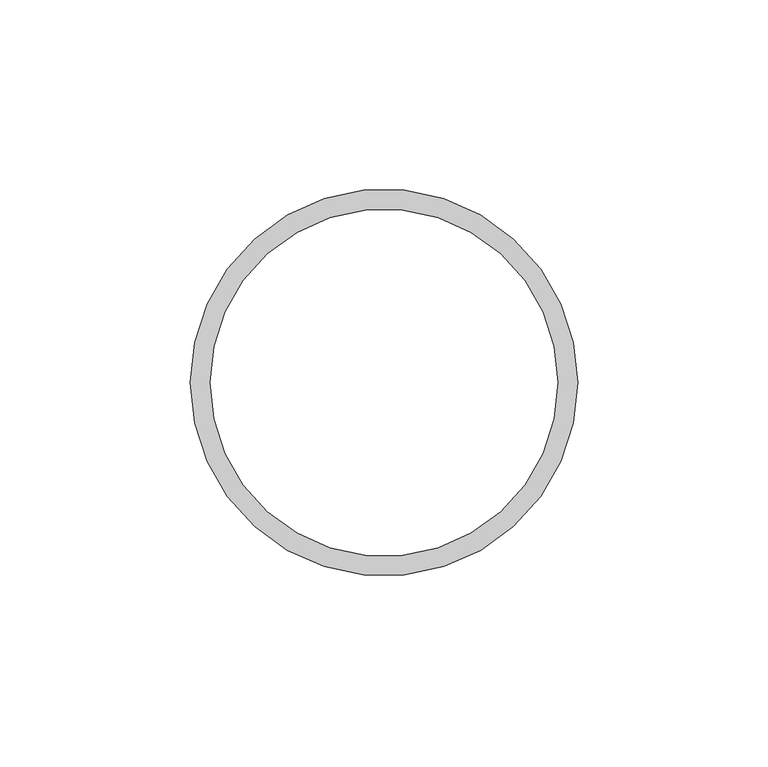
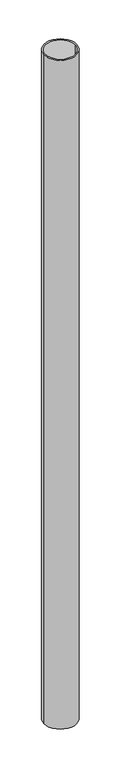
"""IFC4 building model written with IfcOpenShell, lengths in millimetres: proxy geometry, Generic Models 7:Generic Models 1:3:Generic Models 1:3 : Generic Models 7:Generic Models 1:305549:3:Generic Models 1:3:Generic Models 1:3 : Generic Models 7:Generic Models 1:305549:3 : Generic Models 7:Generic Models 1:3:Generic Models 1:3 : Generic Models 7:Generic Models 1:305549:301244:28 : Generic Models 7:Generic Models 1:3:Generic Models 1:3 : Generic Models 7:Generic Models 1:305549:3:Generic Models 1:3:Generic Models 1:3 : Generic Models 7:Generic Models 1:305549:3 : Generic Models 7:Generic Models 1:3:Generic Models 1:3 : Generic Models 7:Generic Models 1:305549:301244:308848."""

from ifc_helpers import new_model, si_unit, point, frame, frame_2d, origin, place, context, project, spatial, circle_curve, trimmed, segment, composite_curve, outline, extrude, source, transform, mapped, element, save


def generic_models_a17a7060(model_context):
    return source(origin(), model_context, "Body", "SweptSolid", [
        extrude(outline(composite_curve([segment(trimmed(circle_curve(frame_2d((560568.8617239, -572593.5413841)), 50.8), [point((560518.0617239, -572593.5413841))], [point((560619.6617239, -572593.5413841))], False, "CARTESIAN"), True, "CONTINUOUS"), segment(trimmed(circle_curve(frame_2d((560568.8617239, -572593.5413841)), 50.8), [point((560619.6617239, -572593.5413841))], [point((560518.0617239, -572593.5413841))], False, "CARTESIAN"), True, "CONTINUOUS")], self_intersect=False), holes=[composite_curve([segment(trimmed(circle_curve(frame_2d((560568.8617239, -572593.5413841)), 45.593), [point((560523.2687239, -572593.5413841))], [point((560614.4547239, -572593.5413841))], True, "CARTESIAN"), True, "CONTINUOUS"), segment(trimmed(circle_curve(frame_2d((560568.8617239, -572593.5413841)), 45.593), [point((560614.4547239, -572593.5413841))], [point((560523.2687239, -572593.5413841))], True, "CARTESIAN"), True, "CONTINUOUS")], self_intersect=False)]), frame((0.0, 0.0, 3929.0269064), z_axis=(0.0, 0.0, 1.0), x_axis=(1.0, 0.0, 0.0)), (0.0, 0.0, 1.0), 2205.0730936),
    ])


if __name__ == "__main__":
    model = new_model("IFC4")
    model_context = context("Model", 3, world=origin())
    ifc_project = project(units=[si_unit("LENGTHUNIT", "METRE", prefix="MILLI")], contexts=[model_context])
    site = spatial("IfcSite", under=ifc_project)
    building = spatial("IfcBuilding", under=site)
    placement = place(None, origin())
    generic_models_shape = generic_models_a17a7060(model_context)
    element("IfcBuildingElementProxy", 1, Name="Generic Models 7:Generic Models 1:3:Generic Models 1:3 : Generic Models 7:Generic Models 1:305549:3:Generic Models 1:3:Generic Models 1:3 : Generic Models 7:Generic Models 1:305549:3 : Generic Models 7:Generic Models 1:3:Generic Models 1:3 : Generic Models 7:Generic Models 1:305549:301244:28 : Generic Models 7:Generic Models 1:3:Generic Models 1:3 : Generic Models 7:Generic Models 1:305549:3:Generic Models 1:3:Generic Models 1:3 : Generic Models 7:Generic Models 1:305549:3 : Generic Models 7:Generic Models 1:3:Generic Models 1:3 : Generic Models 7:Generic Models 1:305549:301244:308848", ObjectType="Generic Models 7:Generic Models 1:3:Generic Models 1:3 : Generic Models 7:Generic Models 1:305549:3:Generic Models 1:3:Generic Models 1:3 : Generic Models 7:Generic Models 1:305549:3 : Generic Models 7:Generic Models 1:3:Generic Models 1:3 : Generic Models 7:Generic Models 1:305549:301244:28 : Generic Models 7:Generic Models 1:3:Generic Models 1:3 : Generic Models 7:Generic Models 1:305549:3:Generic Models 1:3:Generic Models 1:3 : Generic Models 7:Generic Models 1:305549:3 : Generic Models 7:Generic Models 1:3:Generic Models 1:3 : Generic Models 7:Generic Models 1:305549:301244:308848", at=placement, inside=building, context=model_context, shape_type="MappedRepresentation", body=[
        mapped(generic_models_shape, transform((0.0, 0.0, 0.0), x_axis=(1.0, 0.0, 0.0), y_axis=(0.0, 1.0, 0.0), z_axis=(0.0, 0.0, 1.0))),
    ])
    save(model, "model.ifc")

# Revit data of these elements
# Type "Generic Models 7:Generic Models 1:3:Generic Models 1:3 : Generic Models 7:Generic Models 1:305549:3:Generic Models 1:3:Generic Models 1:3 : Generic Models 7:Generic Models 1:305549:3 : Generic Models 7:Generic Models 1:3:Generic Models 1:3 : Generic Models 7:Generic Models 1:305549:301244:28 : Generic Models 7:Generic Models 1:3:Generic Models 1:3 : Generic Models 7:Generic Models 1:305549:3:Generic Models 1:3:Generic Models 1:3 : Generic Models 7:Generic Models 1:305549:3 : Generic Models 7:Generic Models 1:3:Generic Models 1:3 : Generic Models 7:Generic Models 1:305549:301244:308848"
#   NameOverride = "Generic Models 7:Generic Models 1:3:Generic Models 1:3 : Generic Models 7:Generic Models 1:305549:3:Generic Models 1:3:Generic Models 1:3 : Generic Models 7:Generic Models 1:305549:3 : Generic Models 7:Generic Models 1:3:Generic Models 1:3 : Generic Models 7:Generic Models 1:305549:301244:308848"
#   ObjectTypeOverride = "Generic Models 1:3:Generic Models 1:3 : Generic Models 7:Generic Models 1:305549:3 : Generic Models 7:Generic Models 1:3:Generic Models 1:3 : Generic Models 7:Generic Models 1:305549:301244"
#   Reference = "Generic Models 1"
#   Tag = "308848"
